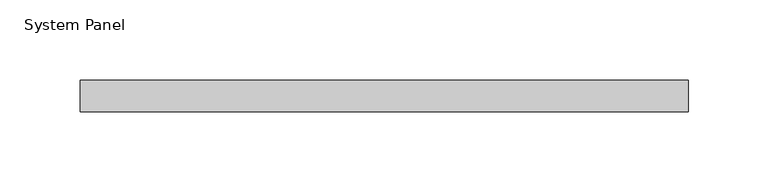
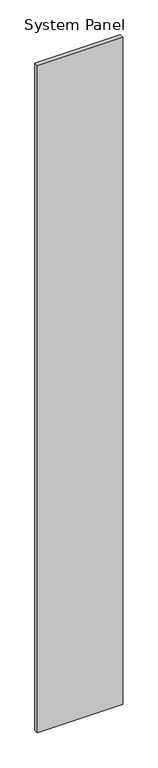
"""IFC4 building model written with IfcOpenShell, lengths in millimetres: plate geometry, System Panel : WWm-Glass-20mm-10mmOffset."""

from ifc_helpers import new_model, si_unit, origin, origin_with_axes, place, context, project, spatial, polyline, outline, extrude, source, transform, mapped, element, save


def system_panel_2693c075(model_context):
    return source(origin(), model_context, "Body", "SweptSolid", [
        extrude(outline(polyline([(190.0, 0.0), (-190.0, 0.0), (-190.0, 20.0), (190.0, 20.0), (190.0, 0.0)])), origin_with_axes(), (0.0, 0.0, 1.0), 3150.0),
    ])


if __name__ == "__main__":
    model = new_model("IFC4")
    model_context = context("Model", 3, world=origin())
    ifc_project = project(units=[si_unit("LENGTHUNIT", "METRE", prefix="MILLI")], contexts=[model_context])
    site = spatial("IfcSite", under=ifc_project)
    building = spatial("IfcBuilding", under=site)
    placement = place(None, origin())
    system_panel_shape = system_panel_2693c075(model_context)
    element("IfcPlate", 1, ObjectType="System Panel : WWm-Glass-20mm-10mmOffset", at=placement, inside=building, context=model_context, shape_type="MappedRepresentation", body=[
        mapped(system_panel_shape, transform((0.0, 0.0, 0.0), x_axis=(1.0, 0.0, 0.0), y_axis=(0.0, 1.0, 0.0), z_axis=(0.0, 0.0, 1.0))),
    ])
    save(model, "model.ifc")

# Revit data of these elements
# Type "System Panel : WWm-Glass-20mm-10mmOffset"
#   Finish = ""
# Element 1 (IfcPlate, "System Panel : WWm-Glass-20mm-10mmOffset")
#   Materials on its faces: "WW-EC-GL-Storefront"
# Materials
#   "WW-EC-GL-Storefront": class "Glass", colour RGB 236 240 239, transparency 0.85, Description = "Storefront Glass", Cost = 0
